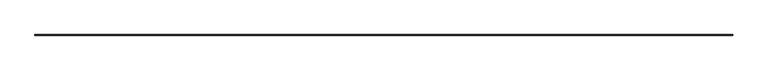
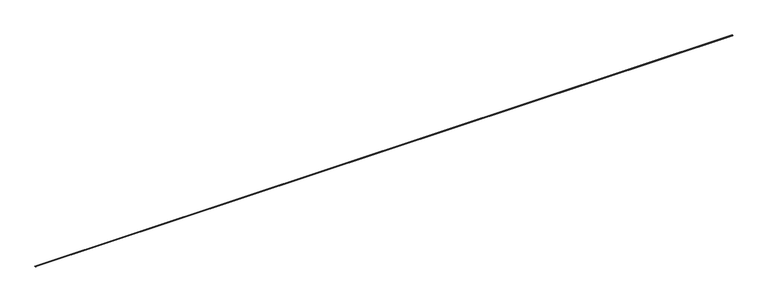
"""IFC4 building model written with IfcOpenShell, lengths in millimetres: proxy geometry, Inner panel:Inner panel:1:Inner panel:1 : Inner panel:Inner panel:300324:2:Inner panel:1:Inner panel:1 : Inner panel:Inner panel:300324:2 : Inner panel:Inner panel:1:Inner panel:1 : Inner panel:Inner panel:300324:300043:45 : Inner panel:Inner panel:1:Inner panel:1 : Inner panel:Inner panel:300324:2:Inner panel:1:Inner panel:1 : Inner panel:Inner panel:300324:2 : Inner panel:Inner panel:1:Inner panel:1 : Inner panel:Inner panel:300324:300043:308120."""

from ifc_helpers import new_model, si_unit, frame, origin, place, context, project, spatial, polyline, outline, extrude, source, transform, mapped, element, save


def generic_models_a445b37c(model_context):
    return source(origin(), model_context, "Body", "SweptSolid", [
        extrude(outline(polyline([(-578927.0334886, 3914.8343718), (-578928.5535239, 3951.3152182), (-578971.4316802, 3949.5286283), (-578969.9116449, 3913.047782), (-578986.5860519, 3912.353015), (-578986.7432925, 3916.126788), (-578985.154415, 3916.126788), (-578985.0660167, 3914.0052273), (-578971.5638572, 3914.5678173), (-578973.0838924, 3951.0486636), (-578927.0334886, 3952.9674304), (-578925.5134534, 3916.4865841), (-578912.0112939, 3917.0491741), (-578912.1024459, 3919.2368232), (-578910.5135685, 3919.2368232), (-578910.3590816, 3915.5291388), (-578927.0334886, 3914.8343718)])), frame((579104.5117239, 0.0, 0.0), z_axis=(1.0, 0.0, 0.0), x_axis=(0.0, 1.0, 0.0)), (0.0, 0.0, 1.0), 88442.8),
    ])


if __name__ == "__main__":
    model = new_model("IFC4")
    model_context = context("Model", 3, world=origin())
    ifc_project = project(units=[si_unit("LENGTHUNIT", "METRE", prefix="MILLI")], contexts=[model_context])
    site = spatial("IfcSite", under=ifc_project)
    building = spatial("IfcBuilding", under=site)
    placement = place(None, origin())
    generic_models_shape = generic_models_a445b37c(model_context)
    element("IfcBuildingElementProxy", 1, Name="Inner panel:Inner panel:1:Inner panel:1 : Inner panel:Inner panel:300324:2:Inner panel:1:Inner panel:1 : Inner panel:Inner panel:300324:2 : Inner panel:Inner panel:1:Inner panel:1 : Inner panel:Inner panel:300324:300043:45 : Inner panel:Inner panel:1:Inner panel:1 : Inner panel:Inner panel:300324:2:Inner panel:1:Inner panel:1 : Inner panel:Inner panel:300324:2 : Inner panel:Inner panel:1:Inner panel:1 : Inner panel:Inner panel:300324:300043:308120", ObjectType="Inner panel:Inner panel:1:Inner panel:1 : Inner panel:Inner panel:300324:2:Inner panel:1:Inner panel:1 : Inner panel:Inner panel:300324:2 : Inner panel:Inner panel:1:Inner panel:1 : Inner panel:Inner panel:300324:300043:45 : Inner panel:Inner panel:1:Inner panel:1 : Inner panel:Inner panel:300324:2:Inner panel:1:Inner panel:1 : Inner panel:Inner panel:300324:2 : Inner panel:Inner panel:1:Inner panel:1 : Inner panel:Inner panel:300324:300043:308120", at=placement, inside=building, context=model_context, shape_type="MappedRepresentation", body=[
        mapped(generic_models_shape, transform((0.0, 0.0, 0.0), x_axis=(1.0, 0.0, 0.0), y_axis=(0.0, 1.0, 0.0), z_axis=(0.0, 0.0, 1.0))),
    ])
    save(model, "model.ifc")

# Revit data of these elements
# Type "Inner panel:Inner panel:1:Inner panel:1 : Inner panel:Inner panel:300324:2:Inner panel:1:Inner panel:1 : Inner panel:Inner panel:300324:2 : Inner panel:Inner panel:1:Inner panel:1 : Inner panel:Inner panel:300324:300043:45 : Inner panel:Inner panel:1:Inner panel:1 : Inner panel:Inner panel:300324:2:Inner panel:1:Inner panel:1 : Inner panel:Inner panel:300324:2 : Inner panel:Inner panel:1:Inner panel:1 : Inner panel:Inner panel:300324:300043:308120"
#   NameOverride = "Inner panel:Inner panel:1:Inner panel:1 : Inner panel:Inner panel:300324:2:Inner panel:1:Inner panel:1 : Inner panel:Inner panel:300324:2 : Inner panel:Inner panel:1:Inner panel:1 : Inner panel:Inner panel:300324:300043:308120"
#   ObjectTypeOverride = "Inner panel:1:Inner panel:1 : Inner panel:Inner panel:300324:2 : Inner panel:Inner panel:1:Inner panel:1 : Inner panel:Inner panel:300324:300043"
#   Reference = "Inner panel"
#   Tag = "308120"
# Element 1 (IfcBuildingElementProxy, "Inner panel:Inner panel:1:Inner panel:1 : Inner panel:Inner panel:300324:2:Inner panel:1:Inner panel:1 : Inner panel:Inner panel:300324:2 : Inner panel:Inner panel:1:Inner panel:1 : Inner panel:Inner panel:300324:300043:45 : Inner panel:Inner panel:1:Inner panel:1 : Inner panel:Inner panel:300324:2:Inner panel:1:Inner panel:1 : Inner panel:Inner panel:300324:2 : Inner panel:Inner panel:1:Inner panel:1 : Inner panel:Inner panel:300324:300043:308120")
#   Materials on its faces: "1 1/2\" HAT CHANNELS - SEE STRUCT. DWGs"
# Materials
#   "1 1/2\" HAT CHANNELS - SEE STRUCT. DWGs": class "Metal", colour RGB 189 187 185, transparency 0, Description = "Structural steel 50ksi", Cost = 0
